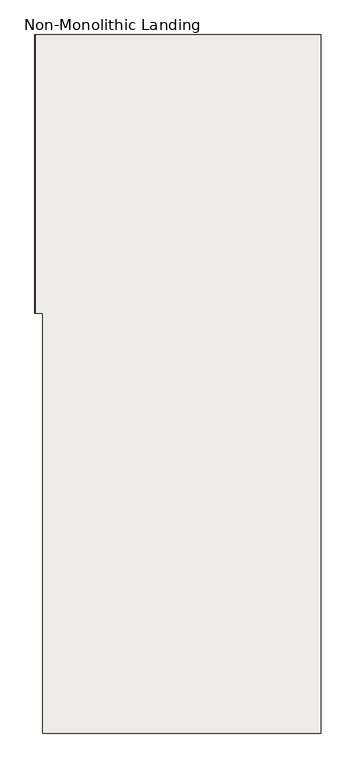
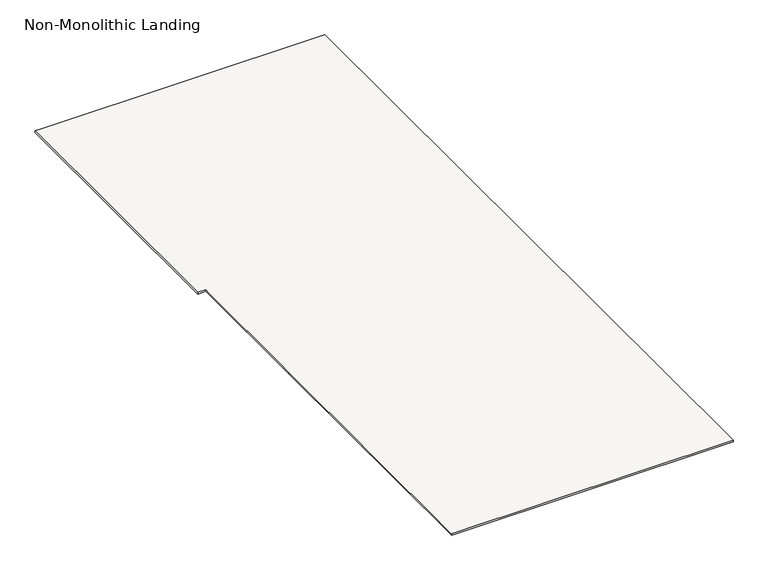
"""IFC4 building model written with IfcOpenShell, lengths in millimetres: slab geometry, Non-Monolithic Landing."""

from ifc_helpers import new_model, si_unit, origin, place, context, project, spatial, faceted_brep, source, transform, mapped, element, save


def non_monolithic_landing_a01bb315(model_context):
    return source(origin(), model_context, "Body", "Brep", [
        faceted_brep([(16318.9409643, 13130.4345331, 1955.5555556), (16318.0972143, 13130.4345331, 1949.5555556), (16318.0972143, 12030.4345331, 1949.5555556), (16318.9409643, 12030.4345331, 1955.5555556), (16350.0, 10370.4345331, 1955.5555556), (17450.0, 10370.4345331, 1955.5555556), (17450.0, 13130.4345331, 1955.5555556), (16350.0, 13130.4345331, 1955.5555556), (16350.0, 12030.4345331, 1955.5555556), (16350.0, 11470.4345331, 1955.5555556), (17450.0, 13130.4345331, 1949.5555556), (17450.0, 10370.4345331, 1949.5555556), (16350.84375, 10370.4345331, 1949.5555556), (16350.84375, 11470.4345331, 1949.5555556), (16350.0, 11470.4345331, 1949.5555556), (16350.0, 12030.4345331, 1949.5555556), (16350.0, 13130.4345331, 1949.5555556)], [[[0, 1, 2, 3]], [[4, 5, 6, 7, 0, 3, 8, 9]], [[10, 11, 12, 13, 14, 15, 2, 1, 16]], [[9, 8, 15, 14]], [[0, 7, 16, 1]], [[7, 6, 10, 16]], [[6, 5, 11, 10]], [[5, 4, 12, 11]], [[13, 9, 14]], [[9, 13, 12, 4]], [[8, 3, 2, 15]]]),
    ])


if __name__ == "__main__":
    model = new_model("IFC4")
    model_context = context("Model", 3, world=origin())
    ifc_project = project(units=[si_unit("LENGTHUNIT", "METRE", prefix="MILLI")], contexts=[model_context])
    site = spatial("IfcSite", under=ifc_project)
    building = spatial("IfcBuilding", under=site)
    placement = place(None, origin())
    non_monolithic_landing_shape = non_monolithic_landing_a01bb315(model_context)
    element("IfcSlab", 1, ObjectType="Non-Monolithic Landing", at=placement, inside=building, context=model_context, shape_type="MappedRepresentation", body=[
        mapped(non_monolithic_landing_shape, transform((0.0, 0.0, 0.0), x_axis=(1.0, 0.0, 0.0), y_axis=(0.0, 1.0, 0.0), z_axis=(0.0, 0.0, 1.0))),
    ])
    save(model, "model.ifc")

# Revit data of these elements
# Element 1 (IfcSlab, "Non-Monolithic Landing")
#   Materials on its faces: "Steel, Paint Finish, Dark Gray"
# Materials
#   "Steel, Paint Finish, Dark Gray": class "Metal", colour RGB 89 89 89, transparency 0, Description = "Steel, paint finish, dark gray, glossy", Cost = 0
